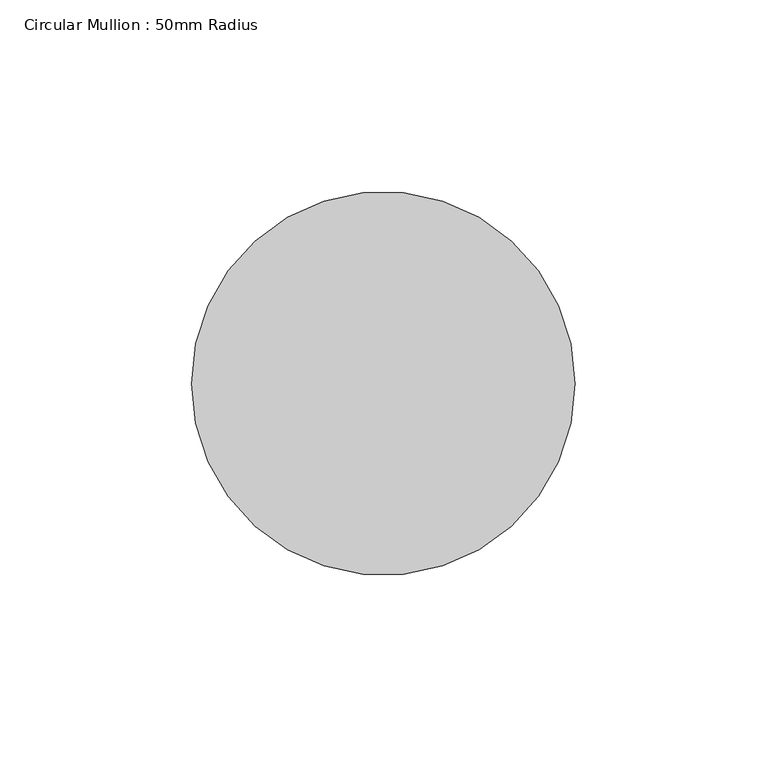
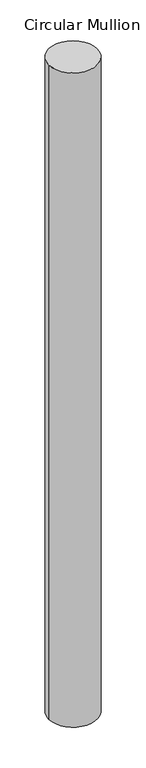
"""IFC4 building model written with IfcOpenShell, lengths in millimetres: member geometry, Circular Mullion : 50mm Radius."""

from ifc_helpers import new_model, si_unit, point, frame, origin, origin_2d, place, context, project, spatial, circle_curve, trimmed, segment, composite_curve, outline, extrude, source, transform, mapped, element, save


def circular_mullion_50mm_radius_e5af3083(model_context):
    return source(origin(), model_context, "Body", "SweptSolid", [
        extrude(outline(composite_curve([segment(trimmed(circle_curve(origin_2d(), 50.0), [point((50.0, 0.0))], [point((-50.0, 0.0))], False, "CARTESIAN"), True, "CONTINUOUS"), segment(trimmed(circle_curve(origin_2d(), 50.0), [point((-50.0, 0.0))], [point((50.0, 0.0))], False, "CARTESIAN"), True, "CONTINUOUS")], self_intersect=False)), frame((0.0, 0.0, -1425.2878908), z_axis=(0.0, 0.0, 1.0), x_axis=(1.0, 0.0, 0.0)), (0.0, 0.0, 1.0), 1425.2878908),
    ])


if __name__ == "__main__":
    model = new_model("IFC4")
    model_context = context("Model", 3, world=origin())
    ifc_project = project(units=[si_unit("LENGTHUNIT", "METRE", prefix="MILLI")], contexts=[model_context])
    site = spatial("IfcSite", under=ifc_project)
    building = spatial("IfcBuilding", under=site)
    placement = place(None, origin())
    circular_mullion_50mm_radius_shape = circular_mullion_50mm_radius_e5af3083(model_context)
    element("IfcMember", 1, ObjectType="Circular Mullion : 50mm Radius", at=placement, inside=building, context=model_context, shape_type="MappedRepresentation", body=[
        mapped(circular_mullion_50mm_radius_shape, transform((0.0, 0.0, 0.0), x_axis=(1.0, 0.0, 0.0), y_axis=(0.0, 1.0, 0.0), z_axis=(0.0, 0.0, 1.0))),
    ])
    save(model, "model.ifc")

# Revit data of these elements
# Type "Circular Mullion : 50mm Radius"
#   built-in parameter 1007350 = 0.164042 (stored number, unit not read)
# Element 1 (IfcMember, "Circular Mullion : 50mm Radius")
#   Materials on its faces: "Aluminium"
# Materials
#   "Aluminium": class "Metal", colour RGB 247 247 247, transparency 0, Description = "Aluminium 6061", Cost = 0
